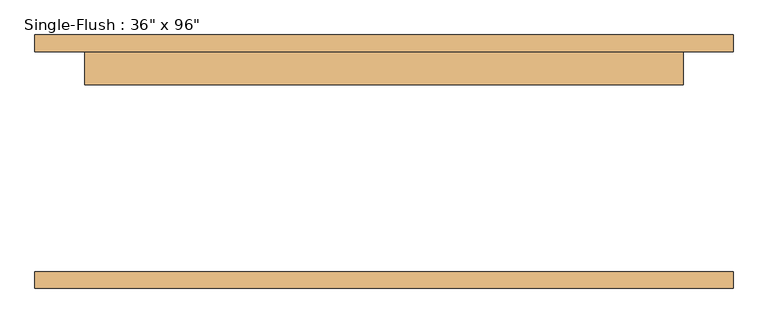
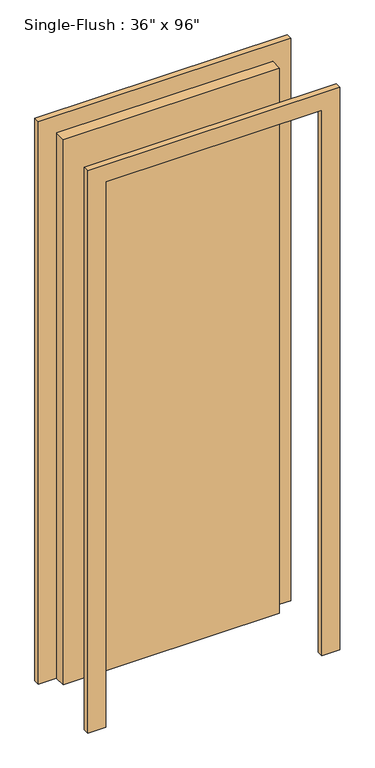
"""IFC4 building model written with IfcOpenShell, lengths in millimetres: door geometry."""

from ifc_helpers import new_model, si_unit, frame, origin, origin_with_axes, place, context, project, spatial, polyline, outline, extrude, source, transform, mapped, element, save


def door_886b15f6(model_context):
    return source(origin(), model_context, "Body", "SweptSolid", [
        extrude(outline(polyline([(2514.6, -533.4), (0.0, -533.4), (0.0, -457.2), (2438.4, -457.2), (2438.4, 457.2), (0.0, 457.2), (0.0, 533.4), (2514.6, 533.4), (2514.6, -533.4)])), frame((0.0, 168.275, 0.0), z_axis=(0.0, 1.0, 0.0), x_axis=(0.0, 0.0, 1.0)), (0.0, 0.0, 1.0), 25.4),
        extrude(outline(polyline([(2514.6, 533.4), (2514.6, -533.4), (0.0, -533.4), (0.0, -457.2), (2438.4, -457.2), (2438.4, 457.2), (0.0, 457.2), (0.0, 533.4), (2514.6, 533.4)])), frame((0.0, -193.675, 0.0), z_axis=(0.0, 1.0, 0.0), x_axis=(0.0, 0.0, 1.0)), (0.0, 0.0, 1.0), 25.4),
        extrude(outline(polyline([(457.2, 117.475), (-457.2, 117.475), (-457.2, 168.275), (457.2, 168.275), (457.2, 117.475)])), origin_with_axes(), (0.0, 0.0, 1.0), 2438.4),
    ])


if __name__ == "__main__":
    model = new_model("IFC4")
    model_context = context("Model", 3, world=origin())
    ifc_project = project(units=[si_unit("LENGTHUNIT", "METRE", prefix="MILLI")], contexts=[model_context])
    site = spatial("IfcSite", under=ifc_project)
    building = spatial("IfcBuilding", under=site)
    placement = place(None, origin())
    door_shape = door_886b15f6(model_context)
    element("IfcDoor", 1, ObjectType="Single-Flush : 36\" x 96\"", at=placement, inside=building, context=model_context, shape_type="MappedRepresentation", body=[
        mapped(door_shape, transform((0.0, 0.0, 0.0), x_axis=(1.0, 0.0, 0.0), y_axis=(0.0, 1.0, 0.0), z_axis=(0.0, 0.0, 1.0))),
    ])
    save(model, "model.ifc")

# Revit data of these elements
# Type "Single-Flush : 36\" x 96\""
#   Type Mark = "32"
#   Construction Type Id = "MDOOR"
#   Assembly Code = "C1020"
#   Analytic Construction = "Metal"
#   Thickness = 0' - 2"
#   Heat Transfer Coefficient (U) = 3.7021 W/(m²·K)
#   Height = 8' - 0"
#   Trim Projection Ext = 0' - 1"
#   Trim Projection Int = 0' - 1"
#   Trim Width = 0' - 3"
#   Width = 3' - 0"
#   Door Material = INTERIOR GRADE ALUMINUM STOREFRONT W/ SAFETY GLAZING
#   Frame Material = INTERIOR GRADE ALUMINUM STOREFRONT W/ SAFETY GLAZING
#   Visual Light Transmittance = 0
#   Solar Heat Gain Coefficient = 0
#   Function = (empty or 0)
#   Wall Closure = (empty or 0)
# Element 1 (IfcDoor, "Single-Flush : 36\" x 96\"")
#   Materials on its faces: "INTERIOR GRADE ALUMINUM STOREFRONT W/ SAFETY GLAZING"
# Materials
#   "INTERIOR GRADE ALUMINUM STOREFRONT W/ SAFETY GLAZING": class "Metal", colour RGB 226 226 226, transparency 0, Description = "Aluminum 6061", Cost = 0
